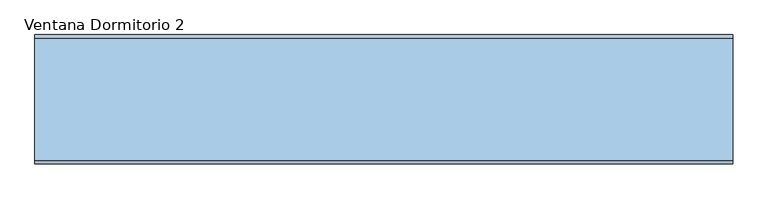
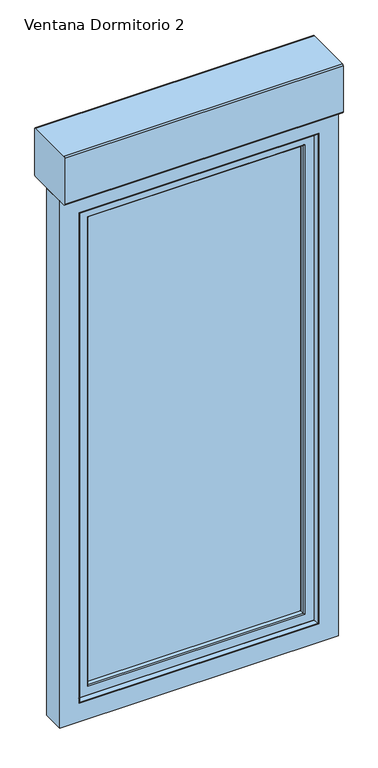
"""IFC4 building model written with IfcOpenShell, lengths in millimetres: window geometry, 2019_ES_Ventana_Replus_re80pvc301_10100_box_1-Hoja_con-Compacto : Ventana Dormitorio 2."""

from ifc_helpers import new_model, si_unit, point, frame, frame_2d, origin, place, context, project, spatial, polyline, circle_curve, ellipse_curve, trimmed, segment, composite_curve, outline, extrude, source, transform, mapped, element, save
from ifc_brep_helpers import plane_surface, cylinder_surface, advanced_brep


def ventana_dormitorio_2_12c73b47(model_context):
    return source(origin(), model_context, "Body", "SolidModel", [
        extrude(outline(composite_curve([segment(trimmed(circle_curve(frame_2d((-55.0, 2815.0)), 5.0), [point((-55.0, 2810.0))], [point((-60.0, 2815.0))], False, "CARTESIAN"), True, "CONTINUOUS"), segment(polyline([(-60.0, 2815.0), (-60.0, 2990.0)]), True, "CONTINUOUS"), segment(trimmed(circle_curve(frame_2d((-55.0, 2990.0)), 5.0), [point((-60.0, 2990.0))], [point((-55.0, 2995.0))], False, "CARTESIAN"), True, "CONTINUOUS"), segment(polyline([(-55.0, 2995.0), (120.0, 2995.0)]), True, "CONTINUOUS"), segment(trimmed(circle_curve(frame_2d((120.0, 2990.0)), 5.0), [point((120.0, 2995.0))], [point((125.0, 2990.0))], False, "CARTESIAN"), True, "CONTINUOUS"), segment(polyline([(125.0, 2990.0), (125.0, 2815.0)]), True, "CONTINUOUS"), segment(trimmed(circle_curve(frame_2d((120.0, 2815.0)), 5.0), [point((125.0, 2815.0))], [point((120.0, 2810.0))], False, "CARTESIAN"), True, "CONTINUOUS"), segment(polyline([(120.0, 2810.0), (-55.0, 2810.0)]), True, "CONTINUOUS")], self_intersect=False)), frame((-500.0, 0.0, 0.0), z_axis=(1.0, 0.0, 0.0), x_axis=(0.0, 1.0, 0.0)), (0.0, 0.0, 1.0), 1000.0),
        extrude(outline(polyline([(78.4999991, 1470.0), (118.4999991, 1470.0), (118.4999991, 1360.0), (98.4999991, 1360.0), (98.4999991, 1450.0), (78.4999991, 1450.0), (78.4999991, 1470.0)])), frame((-434.1999993, 0.0, 0.0), z_axis=(1.0, 0.0, 0.0), x_axis=(0.0, 1.0, 0.0)), (0.0, 0.0, 1.0), 12.0),
        extrude(outline(polyline([(-413.9687607, 78.4999991), (-413.9687607, 68.4999991), (-442.4312378, 68.4999991), (-442.4312378, 78.4999991), (-413.9687607, 78.4999991)])), frame((0.0, 0.0, 1435.217127), z_axis=(0.0, 0.0, 1.0), x_axis=(1.0, 0.0, 0.0)), (0.0, 0.0, 1.0), 49.565746),
        extrude(outline(polyline([(909.8, 397.1999993), (2707.2, 397.1999993), (2707.2, -397.1999993), (909.8, -397.1999993), (909.8, 397.1999993)]), holes=[polyline([(2699.2, 389.1999993), (917.8, 389.1999993), (917.8, -389.1999993), (2699.2, -389.1999993), (2699.2, 389.1999993)])]), frame((0.0, 10.9999999, 0.0), z_axis=(0.0, 1.0, 0.0), x_axis=(0.0, 0.0, 1.0)), (0.0, 0.0, 1.0), 16.0),
        extrude(outline(polyline([(909.8131934, 397.1868058), (2707.1868066, 397.1868058), (2707.1868066, -397.1868058), (909.8131934, -397.1868058), (909.8131934, 397.1868058)]), holes=[polyline([(2699.2, 389.1999993), (917.8, 389.1999993), (917.8, -389.1999993), (2699.2, -389.1999993), (2699.2, 389.1999993)])]), frame((0.0, 31.0000001, 0.0), z_axis=(0.0, 1.0, 0.0), x_axis=(0.0, 0.0, 1.0)), (0.0, 0.0, 1.0), 16.0),
        extrude(outline(polyline([(397.1999993, 6.9999997), (-397.1999993, 6.9999997), (-397.1999993, 10.9999999), (397.1999993, 10.9999999), (397.1999993, 6.9999997)])), frame((0.0, 0.0, 903.7946451), z_axis=(0.0, 0.0, 1.0), x_axis=(1.0, 0.0, 0.0)), (0.0, 0.0, 1.0), 1809.4053549),
        extrude(outline(polyline([(397.1999993, 26.9999999), (-397.1999993, 26.9999999), (-397.1999993, 31.0000001), (397.1999993, 31.0000001), (397.1999993, 26.9999999)])), frame((0.0, 0.0, 903.7946451), z_axis=(0.0, 0.0, 1.0), x_axis=(1.0, 0.0, 0.0)), (0.0, 0.0, 1.0), 1809.4053549),
        extrude(outline(polyline([(397.1999993, 47.0000001), (-397.1999993, 47.0000001), (-397.1999993, 51.0000003), (397.1999993, 51.0000003), (397.1999993, 47.0000001)])), frame((0.0, 0.0, 903.7946451), z_axis=(0.0, 0.0, 1.0), x_axis=(1.0, 0.0, 0.0)), (0.0, 0.0, 1.0), 1809.4053549),
        advanced_brep(
        [(387.2913171, -9.2764571, 2697.2913178), (387.2913171, -9.2764571, 922.7086822), (390.1890946, -11.5, 919.8109047), (390.1890946, -11.5, 2700.1890953), (430.1999993, -11.5, 879.8), (430.1999993, -11.5, 2740.2), (-430.1999993, -11.5, 2740.2), (-430.1999993, -11.5, 879.8), (-390.1890946, -11.5, 919.8109047), (-390.1890946, -11.5, 2700.1890953), (-387.2913171, -9.2764571, 922.7086822), (384.1757968, 2.3508228, 2694.1757976), (384.1757968, 2.3508228, 925.8242024), (-384.1757968, 2.3508228, 925.8242024), (384.6739305, 3.0000033, 2694.6739313), (384.6739305, 3.0000033, 925.3260687), (-384.6739305, 3.0000033, 925.3260687), (391.1999993, 3.0000033, 2701.2), (391.1999993, 3.0000033, 918.8), (-391.1999993, 3.0000033, 918.8), (-391.1999993, 3.0000033, 2701.2), (-384.6739305, 3.0000033, 2694.6739313), (391.1999993, 6.9999997, 2701.2), (391.1999993, 6.9999997, 918.8), (-391.1999993, 6.9999997, 918.8), (411.8162192, 6.9999997, 2721.8162199), (411.8162192, 6.9999997, 898.1837801), (-411.8162192, 6.9999997, 898.1837801), (-411.8162192, 6.9999997, 2721.8162199), (-391.1999993, 6.9999997, 2701.2), (409.1999993, 25.6153717, 2719.2), (409.1999993, 25.6153717, 900.8), (-409.1999993, 25.6153717, 900.8), (409.1999993, 56.4999995, 2719.2), (409.1999993, 56.4999995, 900.8), (-409.1999993, 56.4999995, 900.8), (-409.1999993, 56.4999995, 2719.2), (397.1999993, 56.4999995, 2707.2), (397.1999993, 56.4999995, 912.8), (-397.1999993, 56.4999995, 912.8), (-397.1999993, 56.4999995, 2707.2), (397.1999993, 51.0000003, 2707.2), (397.1999993, 51.0000003, 912.8), (-397.1999993, 51.0000003, 912.8), (-397.1999993, 51.0000003, 2707.2), (386.007687, 51.0000003, 2696.0076877), (386.007687, 51.0000003, 923.9923123), (-386.007687, 51.0000003, 923.9923123), (-386.007687, 51.0000003, 2696.0076877), (385.4940999, 51.6693201, 2695.4941006), (385.4940999, 51.6693201, 924.5058994), (-385.4940999, 51.6693201, 924.5058994), (388.8993918, 64.3780426, 2698.8993925), (388.8993918, 64.3780426, 921.1006075), (-388.8993918, 64.3780426, 921.1006075), (392.6234971, 67.3403297, 2702.6234978), (392.6234971, 67.3403297, 917.3765022), (-392.6234971, 67.3403297, 917.3765022), (405.6488427, 67.7951848, 2715.6488434), (405.6488427, 67.7951848, 904.3511566), (-405.6488427, 67.7951848, 904.3511566), (406.1999993, 67.2629391, 2716.2), (406.1999993, 67.2629391, 903.8), (-406.1999993, 67.2629391, 903.8), (407.4370593, 68.4999991, 2717.43706), (407.4370593, 68.4999991, 902.56294), (-407.4370593, 68.4999991, 902.56294), (460.1999993, 68.4999991, 2770.2), (460.1999993, 68.4999991, 849.8), (-460.1999993, 68.4999991, 849.8), (-460.1999993, 68.4999991, 2770.2), (-407.4370593, 68.4999991, 2717.43706), (463.1999993, 65.4999991, 2773.2), (463.1999993, 65.4999991, 846.8), (-463.1999993, 65.4999991, 846.8), (463.1999993, 50.0, 2773.2), (463.1999993, 50.0, 846.8), (-463.1999993, 50.0, 846.8), (-463.1999993, 50.0, 2773.2), (443.1999993, 50.0, 2753.2), (443.1999993, 50.0, 866.8), (-443.1999993, 50.0, 866.8), (-443.1999993, 50.0, 2753.2), (443.1999993, 11.9999991, 2753.2), (443.1999993, 11.9999991, 866.8), (-443.1999993, 11.9999991, 866.8), (-443.1999993, 11.9999991, 2753.2), (430.1999993, 11.9999991, 2740.2), (430.1999993, 11.9999991, 879.8), (-430.1999993, 11.9999991, 879.8), (-430.1999993, 11.9999991, 2740.2), (-387.2913171, -9.2764571, 2697.2913178), (-384.1757968, 2.3508228, 2694.1757976), (-409.1999993, 25.6153717, 2719.2), (-385.4940999, 51.6693201, 2695.4941006), (-388.8993918, 64.3780426, 2698.8993925), (-392.6234971, 67.3403297, 2702.6234978), (-405.6488427, 67.7951848, 2715.6488434), (-406.1999993, 67.2629391, 2716.2), (-463.1999993, 65.4999991, 2773.2)],
        [
            (0, 1),
            (1, 2, ellipse_curve(frame((390.1890946, -8.5, 919.8109047), z_axis=(0.7071067811865475, 0.0, 0.7071067811865475), x_axis=(-0.7071067811865474, 0.0, 0.7071067811865476)), 4.2426407, 3.0)),
            (2, 3),
            (3, 0, ellipse_curve(frame((390.1890946, -8.5, 2700.1890953), z_axis=(0.7071067811865475, 0.0, -0.7071067811865475), x_axis=(0.7071067811865474, 0.0, 0.7071067811865476)), 4.2426407, 3.0)),
            (4, 5),
            (5, 6),
            (6, 7),
            (7, 4),
            (2, 8),
            (8, 9),
            (9, 3),
            (1, 10),
            (10, 8, ellipse_curve(frame((-390.1890946, -8.5, 919.8109047), z_axis=(0.7071067811865475, 0.0, -0.7071067811865475), x_axis=(0.7071067811865476, 0.0, 0.7071067811865474)), 4.2426407, 3.0)),
            (11, 12),
            (12, 1),
            (0, 11),
            (12, 13),
            (13, 10),
            (14, 15),
            (15, 12, ellipse_curve(frame((384.6739305, 2.4842973, 925.3260687), z_axis=(0.7071067811865475, 0.0, 0.7071067811865475), x_axis=(-0.7071067811865474, 0.0, 0.7071067811865476)), 0.7293184, 0.515706)),
            (11, 14, ellipse_curve(frame((384.6739305, 2.4842973, 2694.6739313), z_axis=(0.7071067811865475, 0.0, -0.7071067811865475), x_axis=(0.7071067811865474, 0.0, 0.7071067811865476)), 0.7293184, 0.515706)),
            (15, 16),
            (16, 13, ellipse_curve(frame((-384.6739305, 2.4842973, 925.3260687), z_axis=(0.7071067811865475, 0.0, -0.7071067811865475), x_axis=(0.7071067811865476, 0.0, 0.7071067811865474)), 0.7293184, 0.515706)),
            (17, 18),
            (18, 19),
            (19, 20),
            (20, 17),
            (14, 21),
            (21, 16),
            (22, 23),
            (23, 18),
            (17, 22),
            (23, 24),
            (24, 19),
            (25, 26),
            (26, 27),
            (27, 28),
            (28, 25),
            (22, 29),
            (29, 24),
            (30, 31),
            (31, 26),
            (25, 30),
            (31, 32),
            (32, 27),
            (33, 34),
            (34, 31),
            (30, 33),
            (34, 35),
            (35, 32),
            (33, 36),
            (36, 35),
            (37, 38),
            (38, 39),
            (39, 40),
            (40, 37),
            (41, 42),
            (42, 38),
            (37, 41),
            (42, 43),
            (43, 39),
            (41, 44),
            (44, 43),
            (45, 46),
            (46, 47),
            (47, 48),
            (48, 45),
            (49, 50),
            (50, 46, ellipse_curve(frame((386.007687, 51.5317048, 923.9923123), z_axis=(0.7071067811865475, 0.0, 0.7071067811865475), x_axis=(-0.7071067811865474, 0.0, 0.7071067811865476)), 0.7519437, 0.5317045)),
            (45, 49, ellipse_curve(frame((386.007687, 51.5317048, 2696.0076877), z_axis=(0.7071067811865475, 0.0, -0.7071067811865475), x_axis=(0.7071067811865474, 0.0, 0.7071067811865476)), 0.7519437, 0.5317045)),
            (50, 51),
            (51, 47, ellipse_curve(frame((-386.007687, 51.5317048, 923.9923123), z_axis=(0.7071067811865475, 0.0, -0.7071067811865475), x_axis=(0.7071067811865476, 0.0, 0.7071067811865474)), 0.7519437, 0.5317045)),
            (52, 53),
            (53, 50),
            (49, 52),
            (53, 54),
            (54, 51),
            (55, 56),
            (56, 53, ellipse_curve(frame((392.7630951, 63.3427664, 917.2369042), z_axis=(0.7071067811865475, 0.0, 0.7071067811865475), x_axis=(-0.7071067811865474, 0.0, 0.7071067811865476)), 5.6568542, 4.0)),
            (52, 55, ellipse_curve(frame((392.7630951, 63.3427664, 2702.7630958), z_axis=(0.7071067811865475, 0.0, -0.7071067811865475), x_axis=(0.7071067811865474, 0.0, 0.7071067811865476)), 5.6568542, 4.0)),
            (56, 57),
            (57, 54, ellipse_curve(frame((-392.7630951, 63.3427664, 917.2369042), z_axis=(0.7071067811865475, 0.0, -0.7071067811865475), x_axis=(0.7071067811865476, 0.0, 0.7071067811865474)), 5.6568542, 4.0)),
            (58, 59),
            (59, 56),
            (55, 58),
            (59, 60),
            (60, 57),
            (61, 62),
            (62, 59, ellipse_curve(frame((405.6674291, 67.2629391, 904.3325701), z_axis=(0.7071067811865475, 0.0, 0.7071067811865475), x_axis=(-0.7071067811865474, 0.0, 0.7071067811865476)), 0.7531679, 0.5325701)),
            (58, 61, ellipse_curve(frame((405.6674291, 67.2629391, 2715.6674299), z_axis=(0.7071067811865475, 0.0, -0.7071067811865475), x_axis=(0.7071067811865474, 0.0, 0.7071067811865476)), 0.7531679, 0.5325701)),
            (62, 63),
            (63, 60, ellipse_curve(frame((-405.6674291, 67.2629391, 904.3325701), z_axis=(0.7071067811865475, 0.0, -0.7071067811865475), x_axis=(0.7071067811865476, 0.0, 0.7071067811865474)), 0.7531679, 0.5325701)),
            (64, 65),
            (65, 62, ellipse_curve(frame((407.4370593, 67.2629391, 902.56294), z_axis=(0.7071067811865475, 0.0, 0.7071067811865475), x_axis=(-0.7071067811865474, 0.0, 0.7071067811865476)), 1.7494671, 1.23706)),
            (61, 64, ellipse_curve(frame((407.4370593, 67.2629391, 2717.43706), z_axis=(0.7071067811865475, 0.0, -0.7071067811865475), x_axis=(0.7071067811865474, 0.0, 0.7071067811865476)), 1.7494671, 1.23706)),
            (65, 66),
            (66, 63, ellipse_curve(frame((-407.4370593, 67.2629391, 902.56294), z_axis=(0.7071067811865475, 0.0, -0.7071067811865475), x_axis=(0.7071067811865476, 0.0, 0.7071067811865474)), 1.7494671, 1.23706)),
            (67, 68),
            (68, 69),
            (69, 70),
            (70, 67),
            (64, 71),
            (71, 66),
            (72, 73),
            (73, 68, ellipse_curve(frame((460.1999993, 65.4999991, 849.8), z_axis=(0.7071067811865475, 0.0, 0.7071067811865475), x_axis=(-0.7071067811865474, 0.0, 0.7071067811865476)), 4.2426407, 3.0)),
            (67, 72, ellipse_curve(frame((460.1999993, 65.4999991, 2770.2), z_axis=(0.7071067811865475, 0.0, -0.7071067811865475), x_axis=(0.7071067811865474, 0.0, 0.7071067811865476)), 4.2426407, 3.0)),
            (73, 74),
            (74, 69, ellipse_curve(frame((-460.1999993, 65.4999991, 849.8), z_axis=(0.7071067811865475, 0.0, -0.7071067811865475), x_axis=(0.7071067811865476, 0.0, 0.7071067811865474)), 4.2426407, 3.0)),
            (75, 76),
            (76, 73),
            (72, 75),
            (76, 77),
            (77, 74),
            (75, 78),
            (78, 77),
            (79, 80),
            (80, 81),
            (81, 82),
            (82, 79),
            (79, 83),
            (83, 84),
            (84, 80),
            (84, 85),
            (85, 81),
            (83, 86),
            (86, 85),
            (87, 88),
            (88, 89),
            (89, 90),
            (90, 87),
            (87, 5),
            (4, 88),
            (7, 89),
            (10, 91),
            (91, 9, ellipse_curve(frame((-390.1890946, -8.5, 2700.1890953), z_axis=(-0.7071067811865475, 0.0, -0.7071067811865475), x_axis=(0.7071067811865474, 0.0, -0.7071067811865476)), 4.2426407, 3.0)),
            (13, 92),
            (92, 91),
            (21, 92, ellipse_curve(frame((-384.6739305, 2.4842973, 2694.6739313), z_axis=(-0.7071067811865475, 0.0, -0.7071067811865475), x_axis=(0.7071067811865474, 0.0, -0.7071067811865476)), 0.7293184, 0.515706)),
            (29, 20),
            (32, 93),
            (93, 28),
            (36, 93),
            (44, 40),
            (51, 94),
            (94, 48, ellipse_curve(frame((-386.007687, 51.5317048, 2696.0076877), z_axis=(-0.7071067811865475, 0.0, -0.7071067811865475), x_axis=(0.7071067811865474, 0.0, -0.7071067811865476)), 0.7519437, 0.5317045)),
            (54, 95),
            (95, 94),
            (57, 96),
            (96, 95, ellipse_curve(frame((-392.7630951, 63.3427664, 2702.7630958), z_axis=(-0.7071067811865475, 0.0, -0.7071067811865475), x_axis=(0.7071067811865474, 0.0, -0.7071067811865476)), 5.6568542, 4.0)),
            (60, 97),
            (97, 96),
            (63, 98),
            (98, 97, ellipse_curve(frame((-405.6674291, 67.2629391, 2715.6674299), z_axis=(-0.7071067811865475, 0.0, -0.7071067811865475), x_axis=(0.7071067811865474, 0.0, -0.7071067811865476)), 0.7531679, 0.5325701)),
            (71, 98, ellipse_curve(frame((-407.4370593, 67.2629391, 2717.43706), z_axis=(-0.7071067811865475, 0.0, -0.7071067811865475), x_axis=(0.7071067811865474, 0.0, -0.7071067811865476)), 1.7494671, 1.23706)),
            (74, 99),
            (99, 70, ellipse_curve(frame((-460.1999993, 65.4999991, 2770.2), z_axis=(-0.7071067811865475, 0.0, -0.7071067811865475), x_axis=(0.7071067811865474, 0.0, -0.7071067811865476)), 4.2426407, 3.0)),
            (78, 99),
            (86, 82),
            (6, 90),
            (91, 0),
            (92, 11),
            (93, 30),
            (94, 49),
            (95, 52),
            (96, 55),
            (97, 58),
            (98, 61),
            (99, 72),
        ],
        [
            cylinder_surface(frame((390.1890946, -8.5, 2773.2), z_axis=(0.0, 0.0, 1.0), x_axis=(-1.0, 0.0, 0.0)), 3.0),
            plane_surface(frame((-430.1999993, -11.5, 2740.2), z_axis=(0.0, -1.0, 0.0), x_axis=(1.0, 0.0, 0.0))),
            cylinder_surface(frame((463.1999993, -8.5, 919.8109047), z_axis=(1.0, 0.0, 0.0), x_axis=(0.0, 0.0, 1.0)), 3.0),
            plane_surface(frame((387.2913171, -9.2764571, 2697.2913178), z_axis=(-0.9659258263570549, -0.2588190448487916, 0.0), x_axis=(0.0, 0.0, -1.0))),
            plane_surface(frame((387.2913171, -9.2764571, 922.7086822), z_axis=(0.0, -0.2588190448487885, 0.9659258263570558), x_axis=(-1.0, 0.0, 0.0))),
            cylinder_surface(frame((384.6739305, 2.4842973, 2773.2), z_axis=(0.0, 0.0, 1.0), x_axis=(-1.0, 0.0, 0.0)), 0.515706),
            cylinder_surface(frame((463.1999993, 2.4842973, 925.3260687), z_axis=(1.0, 0.0, 0.0), x_axis=(0.0, 0.0, 1.0)), 0.515706),
            plane_surface(frame((-384.6739305, 3.0000033, 2694.6739313), z_axis=(0.0, 1.0, 0.0), x_axis=(1.0, 0.0, 0.0))),
            plane_surface(frame((391.1999993, 3.0000033, 2701.2), z_axis=(-1.0, 0.0, 0.0), x_axis=(0.0, 0.0, -1.0))),
            plane_surface(frame((391.1999993, 3.0000033, 918.8), z_axis=(0.0, 0.0, 1.0), x_axis=(-1.0, 0.0, 0.0))),
            plane_surface(frame((-391.1999993, 6.9999997, 2701.2), z_axis=(0.0, 1.0, 0.0), x_axis=(1.0, 0.0, 0.0))),
            plane_surface(frame((411.8162192, 6.9999997, 2721.8162199), z_axis=(-0.9902680687415736, -0.13917310096004265, 0.0), x_axis=(0.0, 0.0, -1.0))),
            plane_surface(frame((411.8162192, 6.9999997, 898.1837801), z_axis=(0.0, -0.13917310096003946, 0.990268068741574), x_axis=(-1.0, 0.0, 0.0))),
            plane_surface(frame((409.1999993, 25.6153717, 2719.2), z_axis=(-1.0, 0.0, 0.0), x_axis=(0.0, 0.0, -1.0))),
            plane_surface(frame((409.1999993, 25.6153717, 900.8), z_axis=(0.0, 0.0, 1.0), x_axis=(-1.0, 0.0, 0.0))),
            plane_surface(frame((-409.1999993, 56.4999995, 2719.2), z_axis=(0.0, -1.0, 0.0), x_axis=(1.0, 0.0, 0.0))),
            plane_surface(frame((397.1999993, 56.4999995, 2707.2), z_axis=(1.0, 0.0, 0.0), x_axis=(0.0, 0.0, -1.0))),
            plane_surface(frame((397.1999993, 56.4999995, 912.8), z_axis=(0.0, 0.0, -1.0), x_axis=(-1.0, 0.0, 0.0))),
            plane_surface(frame((-397.1999993, 51.0000003, 2707.2), z_axis=(0.0, -1.0, 0.0), x_axis=(1.0, 0.0, 0.0))),
            cylinder_surface(frame((386.007687, 51.5317048, 2773.2), z_axis=(0.0, 0.0, 1.0), x_axis=(-1.0, 0.0, 0.0)), 0.5317045),
            cylinder_surface(frame((463.1999993, 51.5317048, 923.9923123), z_axis=(1.0, 0.0, 0.0), x_axis=(0.0, 0.0, 1.0)), 0.5317045),
            plane_surface(frame((385.4940999, 51.6693201, 2695.4941006), z_axis=(-0.9659258262890666, 0.2588190451025272, 0.0), x_axis=(0.0, 0.0, -1.0))),
            plane_surface(frame((385.4940999, 51.6693201, 924.5058994), z_axis=(0.0, 0.2588190451025303, 0.9659258262890658), x_axis=(-1.0, 0.0, 0.0))),
            cylinder_surface(frame((392.7630951, 63.3427664, 2773.2), z_axis=(0.0, 0.0, 1.0), x_axis=(-1.0, 0.0, 0.0)), 4.0),
            cylinder_surface(frame((463.1999993, 63.3427664, 917.2369042), z_axis=(1.0, 0.0, 0.0), x_axis=(0.0, 0.0, 1.0)), 4.0),
            plane_surface(frame((392.6234971, 67.3403297, 2702.6234978), z_axis=(-0.034899496702507804, 0.9993908270190955, 0.0), x_axis=(0.0, 0.0, -1.0))),
            plane_surface(frame((392.6234971, 67.3403297, 917.3765022), z_axis=(0.0, 0.9993908270190957, 0.03489949670250457), x_axis=(-1.0, 0.0, 0.0))),
            cylinder_surface(frame((405.6674291, 67.2629391, 2773.2), z_axis=(0.0, 0.0, 1.0), x_axis=(-1.0, 0.0, 0.0)), 0.5325701),
            cylinder_surface(frame((463.1999993, 67.2629391, 904.3325701), z_axis=(1.0, 0.0, 0.0), x_axis=(0.0, 0.0, 1.0)), 0.5325701),
            cylinder_surface(frame((407.4370593, 67.2629391, 2773.2), z_axis=(0.0, 0.0, 1.0), x_axis=(-1.0, 0.0, 0.0)), 1.23706),
            cylinder_surface(frame((463.1999993, 67.2629391, 902.56294), z_axis=(1.0, 0.0, 0.0), x_axis=(0.0, 0.0, 1.0)), 1.23706),
            plane_surface(frame((-407.4370593, 68.4999991, 2717.43706), z_axis=(0.0, 1.0, 0.0), x_axis=(1.0, 0.0, 0.0))),
            cylinder_surface(frame((460.1999993, 65.4999991, 2773.2), z_axis=(0.0, 0.0, 1.0), x_axis=(-1.0, 0.0, 0.0)), 3.0),
            cylinder_surface(frame((463.1999993, 65.4999991, 849.8), z_axis=(1.0, 0.0, 0.0), x_axis=(0.0, 0.0, 1.0)), 3.0),
            plane_surface(frame((463.1999993, 65.4999991, 2773.2), z_axis=(1.0, 0.0, 0.0), x_axis=(0.0, 0.0, -1.0))),
            plane_surface(frame((463.1999993, 65.4999991, 846.8), z_axis=(0.0, 0.0, -1.0), x_axis=(-1.0, 0.0, 0.0))),
            plane_surface(frame((-459.2000019, 50.0, 2769.2000027), z_axis=(0.0, -1.0, 0.0), x_axis=(1.0, 0.0, 0.0))),
            plane_surface(frame((443.1999993, 45.0999991, 2753.2), z_axis=(1.0, 0.0, 0.0), x_axis=(0.0, 0.0, -1.0))),
            plane_surface(frame((443.1999993, 45.0999991, 866.8), z_axis=(0.0, 0.0, -1.0), x_axis=(-1.0, 0.0, 0.0))),
            plane_surface(frame((-435.7000002, 11.9999991, 2745.7000009), z_axis=(0.0, -1.0, 0.0), x_axis=(1.0, 0.0, 0.0))),
            plane_surface(frame((430.1999993, 1.4999991, 2740.2), z_axis=(1.0, 0.0, 0.0), x_axis=(0.0, 0.0, -1.0))),
            plane_surface(frame((430.1999993, 1.4999991, 879.8), z_axis=(0.0, 0.0, -1.0), x_axis=(-1.0, 0.0, 0.0))),
            cylinder_surface(frame((-390.1890946, -8.5, 846.8), z_axis=(0.0, 0.0, -1.0), x_axis=(1.0, 0.0, 0.0)), 3.0),
            plane_surface(frame((-387.2913171, -9.2764571, 922.7086822), z_axis=(0.9659258263570565, -0.2588190448487853, 0.0), x_axis=(0.0, 0.0, 1.0))),
            cylinder_surface(frame((-384.6739305, 2.4842973, 846.8), z_axis=(0.0, 0.0, -1.0), x_axis=(1.0, 0.0, 0.0)), 0.515706),
            plane_surface(frame((-391.1999993, 3.0000033, 918.8), z_axis=(1.0, 0.0, 0.0), x_axis=(0.0, 0.0, 1.0))),
            plane_surface(frame((-411.8162192, 6.9999997, 898.1837801), z_axis=(0.9902680687415745, -0.13917310096003627, 0.0), x_axis=(0.0, 0.0, 1.0))),
            plane_surface(frame((-409.1999993, 25.6153717, 900.8), z_axis=(1.0, 0.0, 0.0), x_axis=(0.0, 0.0, 1.0))),
            plane_surface(frame((-397.1999993, 56.4999995, 912.8), z_axis=(-1.0, 0.0, 0.0), x_axis=(0.0, 0.0, 1.0))),
            cylinder_surface(frame((-386.007687, 51.5317048, 846.8), z_axis=(0.0, 0.0, -1.0), x_axis=(1.0, 0.0, 0.0)), 0.5317045),
            plane_surface(frame((-385.4940999, 51.6693201, 924.5058994), z_axis=(0.9659258262890649, 0.2588190451025334, 0.0), x_axis=(0.0, 0.0, 1.0))),
            cylinder_surface(frame((-392.7630951, 63.3427664, 846.8), z_axis=(0.0, 0.0, -1.0), x_axis=(1.0, 0.0, 0.0)), 4.0),
            plane_surface(frame((-392.6234971, 67.3403297, 917.3765022), z_axis=(0.03489949670250134, 0.9993908270190958, 0.0), x_axis=(0.0, 0.0, 1.0))),
            cylinder_surface(frame((-405.6674291, 67.2629391, 846.8), z_axis=(0.0, 0.0, -1.0), x_axis=(1.0, 0.0, 0.0)), 0.5325701),
            cylinder_surface(frame((-407.4370593, 67.2629391, 846.8), z_axis=(0.0, 0.0, -1.0), x_axis=(1.0, 0.0, 0.0)), 1.23706),
            cylinder_surface(frame((-460.1999993, 65.4999991, 846.8), z_axis=(0.0, 0.0, -1.0), x_axis=(1.0, 0.0, 0.0)), 3.0),
            plane_surface(frame((-463.1999993, 65.4999991, 846.8), z_axis=(-1.0, 0.0, 0.0), x_axis=(0.0, 0.0, 1.0))),
            plane_surface(frame((-443.1999993, 45.0999991, 866.8), z_axis=(-1.0, 0.0, 0.0), x_axis=(0.0, 0.0, 1.0))),
            plane_surface(frame((-430.1999993, 1.4999991, 879.8), z_axis=(-1.0, 0.0, 0.0), x_axis=(0.0, 0.0, 1.0))),
            cylinder_surface(frame((-463.1999993, -8.5, 2700.1890953), z_axis=(-1.0, 0.0, 0.0), x_axis=(0.0, 0.0, -1.0)), 3.0),
            plane_surface(frame((-387.2913171, -9.2764571, 2697.2913178), z_axis=(0.0, -0.2588190448487885, -0.9659258263570557), x_axis=(1.0, 0.0, 0.0))),
            cylinder_surface(frame((-463.1999993, 2.4842973, 2694.6739313), z_axis=(-1.0, 0.0, 0.0), x_axis=(0.0, 0.0, -1.0)), 0.515706),
            plane_surface(frame((-391.1999993, 3.0000033, 2701.2), z_axis=(0.0, 0.0, -1.0), x_axis=(1.0, 0.0, 0.0))),
            plane_surface(frame((-411.8162192, 6.9999997, 2721.8162199), z_axis=(0.0, -0.13917310096003946, -0.990268068741574), x_axis=(1.0, 0.0, 0.0))),
            plane_surface(frame((-409.1999993, 25.6153717, 2719.2), z_axis=(0.0, 0.0, -1.0), x_axis=(1.0, 0.0, 0.0))),
            plane_surface(frame((-397.1999993, 56.4999995, 2707.2), z_axis=(0.0, 0.0, 1.0), x_axis=(1.0, 0.0, 0.0))),
            cylinder_surface(frame((-463.1999993, 51.5317048, 2696.0076877), z_axis=(-1.0, 0.0, 0.0), x_axis=(0.0, 0.0, -1.0)), 0.5317045),
            plane_surface(frame((-385.4940999, 51.6693201, 2695.4941006), z_axis=(0.0, 0.2588190451025303, -0.9659258262890658), x_axis=(1.0, 0.0, 0.0))),
            cylinder_surface(frame((-463.1999993, 63.3427664, 2702.7630958), z_axis=(-1.0, 0.0, 0.0), x_axis=(0.0, 0.0, -1.0)), 4.0),
            plane_surface(frame((-392.6234971, 67.3403297, 2702.6234978), z_axis=(0.0, 0.9993908270190957, -0.03489949670250457), x_axis=(1.0, 0.0, 0.0))),
            cylinder_surface(frame((-463.1999993, 67.2629391, 2715.6674299), z_axis=(-1.0, 0.0, 0.0), x_axis=(0.0, 0.0, -1.0)), 0.5325701),
            cylinder_surface(frame((-463.1999993, 67.2629391, 2717.43706), z_axis=(-1.0, 0.0, 0.0), x_axis=(0.0, 0.0, -1.0)), 1.23706),
            cylinder_surface(frame((-463.1999993, 65.4999991, 2770.2), z_axis=(-1.0, 0.0, 0.0), x_axis=(0.0, 0.0, -1.0)), 3.0),
            plane_surface(frame((-463.1999993, 65.4999991, 2773.2), z_axis=(0.0, 0.0, 1.0), x_axis=(1.0, 0.0, 0.0))),
            plane_surface(frame((-443.1999993, 45.0999991, 2753.2), z_axis=(0.0, 0.0, 1.0), x_axis=(1.0, 0.0, 0.0))),
            plane_surface(frame((-430.1999993, 1.4999991, 2740.2), z_axis=(0.0, 0.0, 1.0), x_axis=(1.0, 0.0, 0.0))),
        ],
        [
            (0, [[1, 2, 3, 4]]),
            (1, [[5, 6, 7, 8], [-3, 9, 10, 11]]),
            (2, [[12, 13, -9, -2]]),
            (3, [[14, 15, -1, 16]]),
            (4, [[17, 18, -12, -15]]),
            (5, [[19, 20, -14, 21]]),
            (6, [[22, 23, -17, -20]]),
            (7, [[24, 25, 26, 27], [-19, 28, 29, -22]]),
            (8, [[30, 31, -24, 32]]),
            (9, [[33, 34, -25, -31]]),
            (10, [[35, 36, 37, 38], [-30, 39, 40, -33]]),
            (11, [[41, 42, -35, 43]]),
            (12, [[44, 45, -36, -42]]),
            (13, [[46, 47, -41, 48]]),
            (14, [[49, 50, -44, -47]]),
            (15, [[-46, 51, 52, -49], [53, 54, 55, 56]]),
            (16, [[57, 58, -53, 59]]),
            (17, [[60, 61, -54, -58]]),
            (18, [[-57, 62, 63, -60], [64, 65, 66, 67]]),
            (19, [[68, 69, -64, 70]]),
            (20, [[71, 72, -65, -69]]),
            (21, [[73, 74, -68, 75]]),
            (22, [[76, 77, -71, -74]]),
            (23, [[78, 79, -73, 80]]),
            (24, [[81, 82, -76, -79]]),
            (25, [[83, 84, -78, 85]]),
            (26, [[86, 87, -81, -84]]),
            (27, [[88, 89, -83, 90]]),
            (28, [[91, 92, -86, -89]]),
            (29, [[93, 94, -88, 95]]),
            (30, [[96, 97, -91, -94]]),
            (31, [[98, 99, 100, 101], [-93, 102, 103, -96]]),
            (32, [[104, 105, -98, 106]]),
            (33, [[107, 108, -99, -105]]),
            (34, [[109, 110, -104, 111]]),
            (35, [[112, 113, -107, -110]]),
            (36, [[-109, 114, 115, -112], [116, 117, 118, 119]]),
            (37, [[120, 121, 122, -116]]),
            (38, [[123, 124, -117, -122]]),
            (39, [[-121, 125, 126, -123], [127, 128, 129, 130]]),
            (40, [[131, -5, 132, -127]]),
            (41, [[-8, 133, -128, -132]]),
            (42, [[134, 135, -10, -13]]),
            (43, [[136, 137, -134, -18]]),
            (44, [[-29, 138, -136, -23]]),
            (45, [[-40, 139, -26, -34]]),
            (46, [[140, 141, -37, -45]]),
            (47, [[-52, 142, -140, -50]]),
            (48, [[-63, 143, -55, -61]]),
            (49, [[144, 145, -66, -72]]),
            (50, [[146, 147, -144, -77]]),
            (51, [[148, 149, -146, -82]]),
            (52, [[150, 151, -148, -87]]),
            (53, [[152, 153, -150, -92]]),
            (54, [[-103, 154, -152, -97]]),
            (55, [[155, 156, -100, -108]]),
            (56, [[-115, 157, -155, -113]]),
            (57, [[-126, 158, -118, -124]]),
            (58, [[-7, 159, -129, -133]]),
            (59, [[160, -4, -11, -135]]),
            (60, [[161, -16, -160, -137]]),
            (61, [[-28, -21, -161, -138]]),
            (62, [[-39, -32, -27, -139]]),
            (63, [[162, -43, -38, -141]]),
            (64, [[-51, -48, -162, -142]]),
            (65, [[-62, -59, -56, -143]]),
            (66, [[163, -70, -67, -145]]),
            (67, [[164, -75, -163, -147]]),
            (68, [[165, -80, -164, -149]]),
            (69, [[166, -85, -165, -151]]),
            (70, [[167, -90, -166, -153]]),
            (71, [[-102, -95, -167, -154]]),
            (72, [[168, -106, -101, -156]]),
            (73, [[-114, -111, -168, -157]]),
            (74, [[-125, -120, -119, -158]]),
            (75, [[-6, -131, -130, -159]]),
        ],
    ),
        advanced_brep(
        [(423.2673545, -12.758819, 2733.2673545), (423.2673545, -12.758819, 886.7326455), (427.2913185, -27.7764571, 882.7086815), (427.2913185, -27.7764571, 2737.2913185), (430.189096, -30.0, 879.810904), (430.189096, -30.0, 2740.189096), (-423.2673545, -12.758819, 886.7326455), (-427.2913185, -27.7764571, 882.7086815), (424.2332803, -11.5, 2734.2332803), (424.2332803, -11.5, 885.7667197), (500.0, -30.0, 2810.0), (500.0, -30.0, 810.0), (500.0, 50.0, 810.0), (500.0, 50.0, 2810.0), (-500.0, 50.0, 810.0), (-500.0, 50.0, 2810.0), (456.1999993, 50.0, 853.8000007), (456.1999993, 50.0, 2766.1999993), (-456.1999993, 50.0, 2766.1999993), (-456.1999993, 50.0, 853.8000007), (-500.0, -30.0, 810.0), (-500.0, -30.0, 2810.0), (-430.189096, -30.0, 879.810904), (-430.189096, -30.0, 2740.189096), (436.1891471, 8.0, 2746.1891471), (436.1891471, 8.0, 873.8108529), (436.1891471, -11.5, 873.8108529), (436.1891471, -11.5, 2746.1891471), (-436.1891471, -11.5, 873.8108529), (-436.1891471, -11.5, 2746.1891471), (-424.2332803, -11.5, 2734.2332803), (-424.2332803, -11.5, 885.7667197), (-436.1891471, 8.0, 873.8108529), (455.1999993, 8.0, 2765.1999993), (455.1999993, 8.0, 854.8000007), (-455.1999993, 8.0, 854.8000007), (-455.1999993, 8.0, 2765.1999993), (-436.1891471, 8.0, 2746.1891471), (455.1999993, 49.0, 854.8000007), (455.1999993, 49.0, 2765.1999993), (-455.1999993, 49.0, 854.8000007), (-423.2673545, -12.758819, 2733.2673545), (-427.2913185, -27.7764571, 2737.2913185), (-455.1999993, 49.0, 2765.1999993)],
        [
            (0, 1),
            (1, 2),
            (2, 3),
            (3, 0),
            (2, 4, ellipse_curve(frame((430.189096, -27.0, 879.810904), z_axis=(0.7071067811865475, 0.0, 0.7071067811865475), x_axis=(-0.7071067811865474, 0.0, 0.7071067811865476)), 4.2426407, 3.0)),
            (4, 5),
            (5, 3, ellipse_curve(frame((430.189096, -27.0, 2740.189096), z_axis=(0.7071067811865475, 0.0, -0.7071067811865475), x_axis=(0.7071067811865474, 0.0, 0.7071067811865476)), 4.2426407, 3.0)),
            (1, 6),
            (6, 7),
            (7, 2),
            (8, 9),
            (9, 1, ellipse_curve(frame((424.2332803, -12.5, 885.7667197), z_axis=(0.7071067811865475, 0.0, 0.7071067811865475), x_axis=(-0.7071067811865474, 0.0, 0.7071067811865476)), 1.4142136, 1.0)),
            (0, 8, ellipse_curve(frame((424.2332803, -12.5, 2734.2332803), z_axis=(0.7071067811865475, 0.0, -0.7071067811865475), x_axis=(0.7071067811865474, 0.0, 0.7071067811865476)), 1.4142136, 1.0)),
            (10, 11),
            (11, 12),
            (12, 13),
            (13, 10),
            (12, 14),
            (14, 15),
            (15, 13),
            (16, 17),
            (17, 18),
            (18, 19),
            (19, 16),
            (11, 20),
            (20, 14),
            (10, 21),
            (21, 20),
            (4, 22),
            (22, 23),
            (23, 5),
            (24, 25),
            (25, 26),
            (26, 27),
            (27, 24),
            (26, 28),
            (28, 29),
            (29, 27),
            (8, 30),
            (30, 31),
            (31, 9),
            (25, 32),
            (32, 28),
            (33, 34),
            (34, 35),
            (35, 36),
            (36, 33),
            (24, 37),
            (37, 32),
            (16, 38, ellipse_curve(frame((456.1999993, 49.0, 853.8000007), z_axis=(0.7071067811865475, 0.0, 0.7071067811865475), x_axis=(-0.7071067811865474, 0.0, 0.7071067811865476)), 1.4142136, 1.0)),
            (38, 39),
            (39, 17, ellipse_curve(frame((456.1999993, 49.0, 2766.1999993), z_axis=(0.7071067811865475, 0.0, -0.7071067811865475), x_axis=(0.7071067811865474, 0.0, 0.7071067811865476)), 1.4142136, 1.0)),
            (38, 34),
            (33, 39),
            (19, 40, ellipse_curve(frame((-456.1999993, 49.0, 853.8000007), z_axis=(0.7071067811865475, 0.0, -0.7071067811865475), x_axis=(0.7071067811865476, 0.0, 0.7071067811865474)), 1.4142136, 1.0)),
            (40, 38),
            (31, 6, ellipse_curve(frame((-424.2332803, -12.5, 885.7667197), z_axis=(0.7071067811865475, 0.0, -0.7071067811865475), x_axis=(0.7071067811865476, 0.0, 0.7071067811865474)), 1.4142136, 1.0)),
            (7, 22, ellipse_curve(frame((-430.189096, -27.0, 879.810904), z_axis=(0.7071067811865475, 0.0, -0.7071067811865475), x_axis=(0.7071067811865476, 0.0, 0.7071067811865474)), 4.2426407, 3.0)),
            (6, 41),
            (41, 42),
            (42, 7),
            (21, 15),
            (37, 29),
            (40, 35),
            (18, 43, ellipse_curve(frame((-456.1999993, 49.0, 2766.1999993), z_axis=(-0.7071067811865475, 0.0, -0.7071067811865475), x_axis=(0.7071067811865474, 0.0, -0.7071067811865476)), 1.4142136, 1.0)),
            (43, 40),
            (30, 41, ellipse_curve(frame((-424.2332803, -12.5, 2734.2332803), z_axis=(-0.7071067811865475, 0.0, -0.7071067811865475), x_axis=(0.7071067811865474, 0.0, -0.7071067811865476)), 1.4142136, 1.0)),
            (42, 23, ellipse_curve(frame((-430.189096, -27.0, 2740.189096), z_axis=(-0.7071067811865475, 0.0, -0.7071067811865475), x_axis=(0.7071067811865474, 0.0, -0.7071067811865476)), 4.2426407, 3.0)),
            (43, 36),
            (41, 0),
            (3, 42),
            (39, 43),
        ],
        [
            plane_surface(frame((427.2913185, -27.7764571, 2737.2913185), z_axis=(-0.9659258262890693, -0.2588190451025169, 0.0), x_axis=(0.0, 0.0, -1.0))),
            cylinder_surface(frame((430.189096, -27.0, 2810.0), z_axis=(0.0, 0.0, 1.0), x_axis=(-1.0, 0.0, 0.0)), 3.0),
            plane_surface(frame((427.2913185, -27.7764571, 882.7086815), z_axis=(0.0, -0.2588190451025138, 0.9659258262890702), x_axis=(-1.0, 0.0, 0.0))),
            cylinder_surface(frame((424.2332803, -12.5, 2810.0), z_axis=(0.0, 0.0, 1.0), x_axis=(-1.0, 0.0, 0.0)), 1.0),
            plane_surface(frame((500.0, 50.0, 2810.0), z_axis=(1.0, 0.0, 0.0), x_axis=(0.0, 0.0, -1.0))),
            plane_surface(frame((-456.1999993, 50.0, 2766.1999993), z_axis=(0.0, 1.0, 0.0), x_axis=(1.0, 0.0, 0.0))),
            plane_surface(frame((500.0, 50.0, 810.0), z_axis=(0.0, 0.0, -1.0), x_axis=(-1.0, 0.0, 0.0))),
            plane_surface(frame((-500.0, -30.0, 2810.0), z_axis=(0.0, -1.0, 0.0), x_axis=(1.0, 0.0, 0.0))),
            plane_surface(frame((436.1891471, -11.5, 2746.1891471), z_axis=(-1.0, 0.0, 0.0), x_axis=(0.0, 0.0, -1.0))),
            plane_surface(frame((-424.2332803, -11.5, 2734.2332803), z_axis=(0.0, 1.0, 0.0), x_axis=(1.0, 0.0, 0.0))),
            plane_surface(frame((436.1891471, -11.5, 873.8108529), z_axis=(0.0, 0.0, 1.0), x_axis=(-1.0, 0.0, 0.0))),
            plane_surface(frame((-436.1891471, 8.0, 2746.1891471), z_axis=(0.0, 1.0, 0.0), x_axis=(1.0, 0.0, 0.0))),
            cylinder_surface(frame((456.1999993, 49.0, 2810.0), z_axis=(0.0, 0.0, 1.0), x_axis=(-1.0, 0.0, 0.0)), 1.0),
            plane_surface(frame((455.1999993, 8.0, 2765.1999993), z_axis=(-1.0, 0.0, 0.0), x_axis=(0.0, 0.0, -1.0))),
            cylinder_surface(frame((500.0, 49.0, 853.8000007), z_axis=(1.0, 0.0, 0.0), x_axis=(0.0, 0.0, 1.0)), 1.0),
            cylinder_surface(frame((500.0, -12.5, 885.7667197), z_axis=(1.0, 0.0, 0.0), x_axis=(0.0, 0.0, 1.0)), 1.0),
            cylinder_surface(frame((500.0, -27.0, 879.810904), z_axis=(1.0, 0.0, 0.0), x_axis=(0.0, 0.0, 1.0)), 3.0),
            plane_surface(frame((-427.2913185, -27.7764571, 882.7086815), z_axis=(0.9659258262890711, -0.2588190451025107, 0.0), x_axis=(0.0, 0.0, 1.0))),
            plane_surface(frame((-500.0, 50.0, 810.0), z_axis=(-1.0, 0.0, 0.0), x_axis=(0.0, 0.0, 1.0))),
            plane_surface(frame((-436.1891471, -11.5, 873.8108529), z_axis=(1.0, 0.0, 0.0), x_axis=(0.0, 0.0, 1.0))),
            plane_surface(frame((455.1999993, 8.0, 854.8000007), z_axis=(0.0, 0.0, 1.0), x_axis=(-1.0, 0.0, 0.0))),
            cylinder_surface(frame((-456.1999993, 49.0, 810.0), z_axis=(0.0, 0.0, -1.0), x_axis=(1.0, 0.0, 0.0)), 1.0),
            cylinder_surface(frame((-424.2332803, -12.5, 810.0), z_axis=(0.0, 0.0, -1.0), x_axis=(1.0, 0.0, 0.0)), 1.0),
            cylinder_surface(frame((-430.189096, -27.0, 810.0), z_axis=(0.0, 0.0, -1.0), x_axis=(1.0, 0.0, 0.0)), 3.0),
            plane_surface(frame((-455.1999993, 8.0, 854.8000007), z_axis=(1.0, 0.0, 0.0), x_axis=(0.0, 0.0, 1.0))),
            plane_surface(frame((-427.2913185, -27.7764571, 2737.2913185), z_axis=(0.0, -0.2588190451025138, -0.9659258262890702), x_axis=(1.0, 0.0, 0.0))),
            plane_surface(frame((-500.0, 50.0, 2810.0), z_axis=(0.0, 0.0, 1.0), x_axis=(1.0, 0.0, 0.0))),
            plane_surface(frame((-436.1891471, -11.5, 2746.1891471), z_axis=(0.0, 0.0, -1.0), x_axis=(1.0, 0.0, 0.0))),
            cylinder_surface(frame((-500.0, 49.0, 2766.1999993), z_axis=(-1.0, 0.0, 0.0), x_axis=(0.0, 0.0, -1.0)), 1.0),
            cylinder_surface(frame((-500.0, -12.5, 2734.2332803), z_axis=(-1.0, 0.0, 0.0), x_axis=(0.0, 0.0, -1.0)), 1.0),
            cylinder_surface(frame((-500.0, -27.0, 2740.189096), z_axis=(-1.0, 0.0, 0.0), x_axis=(0.0, 0.0, -1.0)), 3.0),
            plane_surface(frame((-455.1999993, 8.0, 2765.1999993), z_axis=(0.0, 0.0, -1.0), x_axis=(1.0, 0.0, 0.0))),
        ],
        [
            (0, [[1, 2, 3, 4]]),
            (1, [[-3, 5, 6, 7]]),
            (2, [[8, 9, 10, -2]]),
            (3, [[11, 12, -1, 13]]),
            (4, [[14, 15, 16, 17]]),
            (5, [[-16, 18, 19, 20], [21, 22, 23, 24]]),
            (6, [[25, 26, -18, -15]]),
            (7, [[-14, 27, 28, -25], [-6, 29, 30, 31]]),
            (8, [[32, 33, 34, 35]]),
            (9, [[-34, 36, 37, 38], [-11, 39, 40, 41]]),
            (10, [[42, 43, -36, -33]]),
            (11, [[44, 45, 46, 47], [-32, 48, 49, -42]]),
            (12, [[-21, 50, 51, 52]]),
            (13, [[-51, 53, -44, 54]]),
            (14, [[-24, 55, 56, -50]]),
            (15, [[-41, 57, -8, -12]]),
            (16, [[-10, 58, -29, -5]]),
            (17, [[59, 60, 61, -9]]),
            (18, [[-28, 62, -19, -26]]),
            (19, [[-49, 63, -37, -43]]),
            (20, [[-56, 64, -45, -53]]),
            (21, [[-23, 65, 66, -55]]),
            (22, [[-40, 67, -59, -57]]),
            (23, [[-61, 68, -30, -58]]),
            (24, [[-66, 69, -46, -64]]),
            (25, [[70, -4, 71, -60]]),
            (26, [[-27, -17, -20, -62]]),
            (27, [[-48, -35, -38, -63]]),
            (28, [[-22, -52, 72, -65]]),
            (29, [[-39, -13, -70, -67]]),
            (30, [[-71, -7, -31, -68]]),
            (31, [[-72, -54, -47, -69]]),
        ],
    ),
    ])


if __name__ == "__main__":
    model = new_model("IFC4")
    model_context = context("Model", 3, world=origin())
    ifc_project = project(units=[si_unit("LENGTHUNIT", "METRE", prefix="MILLI")], contexts=[model_context])
    site = spatial("IfcSite", under=ifc_project)
    building = spatial("IfcBuilding", under=site)
    placement = place(None, origin())
    ventana_dormitorio_2_shape = ventana_dormitorio_2_12c73b47(model_context)
    element("IfcWindow", 1, ObjectType="2019_ES_Ventana_Replus_re80pvc301_10100_box_1-Hoja_con-Compacto : Ventana Dormitorio 2", at=placement, inside=building, context=model_context, shape_type="MappedRepresentation", body=[
        mapped(ventana_dormitorio_2_shape, transform((0.0, 0.0, 0.0), x_axis=(1.0, 0.0, 0.0), y_axis=(0.0, 1.0, 0.0), z_axis=(0.0, 0.0, 1.0))),
    ])
    save(model, "model.ifc")

# Revit data of these elements
# Type "2019_ES_Ventana_Replus_re80pvc301_10100_box_1-Hoja_con-Compacto : Ventana Dormitorio 2"
#   Type Mark = "45"
#   URL = "https://replus.es/"
#   Product data url = "https://bimetica.com/es/objetos-bim-replus-ventana-practicable-oscilobatiente-una-hoja-con-compacto-9540"
#   Product Guid = ""
#   Model = "10100 BOX"
#   Material secondary = "Glass"
#   Material main = "PVC"
#   Manufacturer = "Replus"
#   Keynote = "08500"
#   EAN code = ""
#   Description = "Perfiles de PVC con triple junta (por junta rígida en el marco). Protegiendo de este modo todos los puntos de cierre y proporcionando una junta perimetral completa, con un grosor en el perfil de 3 mm. Vidrio de alta calidad con diferentes posibilidades"
#   Assembly Code = "B2020100"
#   Analytic Construction = "<None>"
#   Ι_Wll Thcknss [instance default] = 20.0 cm
#   Ι_Wdth Cntrl = 100.0 cm
#   Ι_Nst Cntrl [instance default] = 0.0 cm
#   Ι_Hndl Hght Cntrl = 65.0 cm
#   Ι_Hght Cntrl = 200.0 cm
#   Rough Width = 102.0 cm
#   Rough Height = 202.0 cm
#   Retranqueo [instance default] = 0.0 cm
#   I_Lf_Cntrl = 92.64 cm
#   Hueco = 1.0 cm
#   Height = 200.0 cm
#   Default Sill Height = 80.0 cm
#   Width = 100.0 cm
#   Altura de Manilla = 65.0 cm
#   Visibilidad Líneas Apertura - Planta = yes
#   Visibilidad Líneas Apertura - Alzado = yes
#   Exceso Dimensiones = no
#   Edition number = 1
#   Advertencia Dimensión = yes
#   Product Material = PVC - Replus - 9152 - White
#   Wall Closure = (empty or 0)
# Element 1 (IfcWindow, "2019_ES_Ventana_Replus_re80pvc301_10100_box_1-Hoja_con-Compacto : Ventana Dormitorio 2")
#   Ι_Wll Thcknss = 10.0 cm
#   Materials on its faces: "PVC - Replus - 9152 - White", "Rubber - Replus - Black", "Glass - Replus"
# Materials
#   "PVC - Replus - 9152 - White": class "Miscellaneous", colour RGB 174 174 166, transparency 0, Manufacturer = "Replus", Comments = "Rendering appearance not upgraded ", URL = "https://replus.es/", Cost = 0
#   "Rubber - Replus - Black": class "Plastic", colour RGB 63 63 63, transparency 0, Description = "Natural rubber, black", Cost = 0
#   "Glass - Replus": class "Glass", colour RGB 218 227 224, transparency 0.85, Cost = 0
